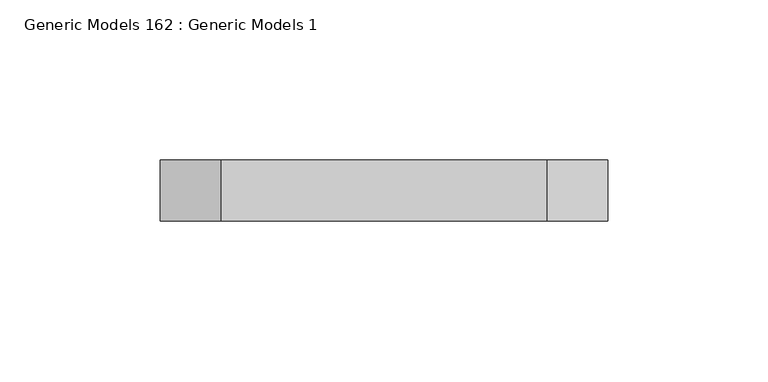
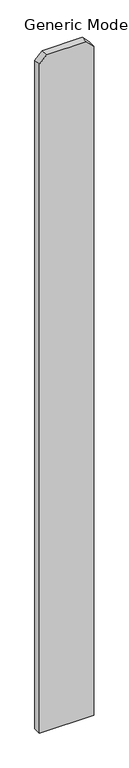
"""IFC4 building model written with IfcOpenShell, lengths in millimetres: proxy geometry, Generic Models 162 : Generic Models 1."""

import ifcopenshell
import ifcopenshell.guid

model = None  # the IFC model being written
_history = None  # IfcOwnerHistory: only IFC2X3 demands one
_inside = {}  # id of a spatial element -> (the spatial element, [elements in it])
_under = {}  # id of a project, library or spatial element -> (it, [spatial elements below it])
_declared = {}  # id of a project -> (the project, [libraries it declares])
_typed = {}  # id of a type object -> (the type object, [elements of that type])
_made_of = {}  # id of a material, layer set ... -> (it, [elements and type objects made of it])


def new_model(schema):
    """Start an empty IFC model of exactly this schema.

    Asked for "IFC4X3", IfcOpenShell would pick the latest addendum, in which some entities
    have other attributes; the version numbers below select the first issue.
    IFC2X3 requires an IfcOwnerHistory on every rooted entity: one is made here for all.
    """
    global model, _history
    if schema == "IFC4X3":
        model = ifcopenshell.file(schema_version=(4, 3, 0, 0))
    else:
        model = ifcopenshell.file(schema=schema)
    _inside.clear()
    _under.clear()
    _declared.clear()
    _typed.clear()
    _made_of.clear()
    _history = None
    if model.schema == "IFC2X3":
        org = make("IfcOrganization", Name="unknown")
        user = make(
            "IfcPersonAndOrganization",
            ThePerson=make("IfcPerson", FamilyName="unknown"),
            TheOrganization=org,
        )
        app = make(
            "IfcApplication",
            ApplicationDeveloper=org,
            Version="unknown",
            ApplicationFullName="unknown",
            ApplicationIdentifier="unknown",
        )
        _history = make(
            "IfcOwnerHistory",
            OwningUser=user,
            OwningApplication=app,
            ChangeAction="ADDED",
            CreationDate=0,
        )
    return model


def make(cls, **values):
    """One entity of the class cls with the attributes given. An attribute that is None is left unset."""
    return model.create_entity(
        cls, **{name: value for name, value in values.items() if value is not None}
    )


def rooted(cls, **values):
    """An entity with a GlobalId (a new one), such as an element, a storey or a relation."""
    return make(cls, GlobalId=ifcopenshell.guid.new(), OwnerHistory=_history, **values)


def si_unit(unit_type, name, prefix=None):
    """IfcSIUnit, for example si_unit("LENGTHUNIT", "METRE", prefix="MILLI")."""
    return make("IfcSIUnit", UnitType=unit_type, Prefix=prefix, Name=name)


def assignment(units):
    """IfcUnitAssignment: the units of a project."""
    return None if units is None else make("IfcUnitAssignment", Units=units)


def point(xyz):
    """IfcCartesianPoint."""
    return None if xyz is None else make("IfcCartesianPoint", Coordinates=xyz)


def direction(xyz):
    """IfcDirection."""
    return None if xyz is None else make("IfcDirection", DirectionRatios=xyz)


def frame(location, z_axis=None, x_axis=None):
    """IfcAxis2Placement3D, a coordinate frame: its origin and axes. An axis left out is left unset."""
    return make(
        "IfcAxis2Placement3D",
        Location=point(location),
        Axis=direction(z_axis),
        RefDirection=direction(x_axis),
    )


def origin():
    """The frame at (0, 0, 0) with its axes left unset."""
    return frame((0.0, 0.0, 0.0))


def place(relative_to, where):
    """IfcLocalPlacement: puts the frame where relative to a parent placement (None: the world)."""
    return make(
        "IfcLocalPlacement", PlacementRelTo=relative_to, RelativePlacement=where
    )


def context(
    kind, dimensions, precision=None, world=None, true_north=None, identifier=None
):
    """IfcGeometricRepresentationContext, for example the 3D "Model" context."""
    return make(
        "IfcGeometricRepresentationContext",
        ContextIdentifier=identifier,
        ContextType=kind,
        CoordinateSpaceDimension=dimensions,
        Precision=precision,
        WorldCoordinateSystem=world,
        TrueNorth=true_north,
    )


def project(units=None, contexts=None):
    """IfcProject with its units and contexts."""
    return rooted(
        "IfcProject",
        Name="project",
        RepresentationContexts=contexts,
        UnitsInContext=assignment(units),
    )


def spatial(cls, under=None, at=None, **own):
    """A site, building, storey or space (cls), placed at a placement, below another one or the project."""
    s = rooted(cls, ObjectPlacement=at, **own)
    if under is not None:
        _under.setdefault(under.id(), (under, []))[1].append(s)
    return s


def polyline(points):
    """IfcPolyline through the points."""
    return make("IfcPolyline", Points=[point(p) for p in points])


def outline(outer, holes=None, kind="AREA"):
    """IfcArbitraryClosedProfileDef: a profile drawn as a closed curve; with holes, ...WithVoids."""
    if holes is None:
        return make("IfcArbitraryClosedProfileDef", ProfileType=kind, OuterCurve=outer)
    return make(
        "IfcArbitraryProfileDefWithVoids",
        ProfileType=kind,
        OuterCurve=outer,
        InnerCurves=holes,
    )


def extrude(swept, where, along, depth):
    """IfcExtrudedAreaSolid: the profile swept, set in the frame where, extruded along a direction by depth."""
    return make(
        "IfcExtrudedAreaSolid",
        SweptArea=swept,
        Position=where,
        ExtrudedDirection=direction(along),
        Depth=depth,
    )


def shape(context_of_items, identifier, shape_type, items):
    """IfcShapeRepresentation: the items that make up one representation, for example the "Body"."""
    return make(
        "IfcShapeRepresentation",
        ContextOfItems=context_of_items,
        RepresentationIdentifier=identifier,
        RepresentationType=shape_type,
        Items=items,
    )


def source(mapping_origin, context_of_items, identifier, shape_type, items):
    """IfcRepresentationMap: a shape defined once, which mapped items show again and again."""
    return make(
        "IfcRepresentationMap",
        MappingOrigin=mapping_origin,
        MappedRepresentation=shape(context_of_items, identifier, shape_type, items),
    )


def transform(
    local_origin,
    x_axis=None,
    y_axis=None,
    z_axis=None,
    scale=None,
    scale2=None,
    scale3=None,
    uniform=True,
):
    """IfcCartesianTransformationOperator3D, or its non-uniform kind. x_axis, y_axis, z_axis: its Axis1, 2, 3."""
    if uniform:
        return make(
            "IfcCartesianTransformationOperator3D",
            Axis1=direction(x_axis),
            Axis2=direction(y_axis),
            LocalOrigin=point(local_origin),
            Scale=scale,
            Axis3=direction(z_axis),
        )
    return make(
        "IfcCartesianTransformationOperator3DnonUniform",
        Axis1=direction(x_axis),
        Axis2=direction(y_axis),
        LocalOrigin=point(local_origin),
        Scale=scale,
        Axis3=direction(z_axis),
        Scale2=scale2,
        Scale3=scale3,
    )


def mapped(mapping_source, mapping_target):
    """IfcMappedItem: shows the shape of a source again, moved by a transform."""
    return make(
        "IfcMappedItem", MappingSource=mapping_source, MappingTarget=mapping_target
    )


def made_of(thing, what):
    """Note that an element or type object is made of a material, layer set ...; save() writes the relation."""
    if what is not None:
        _made_of.setdefault(what.id(), (what, []))[1].append(thing)
    return thing


def element(
    cls,
    number,
    at=None,
    inside=None,
    cuts=None,
    type_object=None,
    material=None,
    context=None,
    identifier="Body",
    shape_type=None,
    held_by="IfcProductDefinitionShape",
    body=None,
    shapes=None,
    **own,
):
    """One element of the class cls, such as IfcWall. Its Tag is "e" and its number.

    at: its placement. inside: the storey or other place that contains it. cuts: it is an
    opening in that element (IfcRelVoidsElement). A single representation is given by context,
    identifier, shape_type and body (its items); several are given by shapes. held_by: the class
    of the entity that holds the representations. save() writes the other relations.
    """
    e = rooted(cls, Tag="e%d" % number, ObjectPlacement=at, **own)
    if body is not None:
        shapes = [shape(context, identifier, shape_type, body)]
    if shapes is not None:
        e.Representation = make(held_by, Representations=shapes)
    if inside is not None:
        _inside.setdefault(inside.id(), (inside, []))[1].append(e)
    if cuts is not None:
        rooted(
            "IfcRelVoidsElement", RelatingBuildingElement=cuts, RelatedOpeningElement=e
        )
    if type_object is not None:
        _typed.setdefault(type_object.id(), (type_object, []))[1].append(e)
    return made_of(e, material)


def aggregate(whole, parts):
    """IfcRelAggregates: a whole, such as a stair, and the parts it consists of."""
    return rooted("IfcRelAggregates", RelatingObject=whole, RelatedObjects=parts)


def save(model, path):
    """Write the relations noted so far, then the file.

    IfcRelAggregates (storeys below a building ...), IfcRelContainedInSpatialStructure (elements
    in a storey), IfcRelDefinesByType, IfcRelAssociatesMaterial and IfcRelDeclares: one each for
    every whole, place, type object, material and project.
    """
    for whole, parts in _under.values():
        aggregate(whole, parts)
    for where, things in _inside.values():
        rooted(
            "IfcRelContainedInSpatialStructure",
            RelatedElements=things,
            RelatingStructure=where,
        )
    for kind, things in _typed.values():
        rooted("IfcRelDefinesByType", RelatedObjects=things, RelatingType=kind)
    for what, things in _made_of.values():
        rooted("IfcRelAssociatesMaterial", RelatedObjects=things, RelatingMaterial=what)
    for by, libraries in _declared.values():
        rooted("IfcRelDeclares", RelatingContext=by, RelatedDefinitions=libraries)
    model.write(path)


def generic_models_162_generic_models_1_9f0ac15c(model_context):
    return source(origin(), model_context, "Body", "SweptSolid", [
        extrude(outline(polyline([(76.2, -250115.3875), (1885.95, -250115.3875), (1905.0, -250134.4375), (1905.0, -250236.0375), (1885.95, -250255.0875), (76.2, -250255.0875), (76.2, -250115.3875)])), frame((0.0, 547.6875, 0.0), z_axis=(0.0, 1.0, 0.0), x_axis=(0.0, 0.0, 1.0)), (0.0, 0.0, 1.0), 19.05),
    ])


if __name__ == "__main__":
    model = new_model("IFC4")
    model_context = context("Model", 3, world=origin())
    ifc_project = project(units=[si_unit("LENGTHUNIT", "METRE", prefix="MILLI")], contexts=[model_context])
    site = spatial("IfcSite", under=ifc_project)
    building = spatial("IfcBuilding", under=site)
    placement = place(None, origin())
    generic_models_162_generic_models_1_shape = generic_models_162_generic_models_1_9f0ac15c(model_context)
    element("IfcBuildingElementProxy", 1, Name="Generic Models 162 : Generic Models 1", ObjectType="Generic Models 162 : Generic Models 1", at=placement, inside=building, context=model_context, shape_type="MappedRepresentation", body=[
        mapped(generic_models_162_generic_models_1_shape, transform((0.0, 0.0, 0.0), x_axis=(1.0, 0.0, 0.0), y_axis=(0.0, 1.0, 0.0), z_axis=(0.0, 0.0, 1.0))),
    ])
    save(model, "model.ifc")

# Revit data of these elements
# Element 1 (IfcBuildingElementProxy, "Generic Models 162 : Generic Models 1")
#   Materials on its faces: "VERTICAL 1X6 CEDAR PLANKS W/ CLEAR WOOD SEALER"
# Materials
#   "VERTICAL 1X6 CEDAR PLANKS W/ CLEAR WOOD SEALER": class "Wood", colour RGB 234 198 147, transparency 0, Description = "Pinus Echinata", Cost = 0
